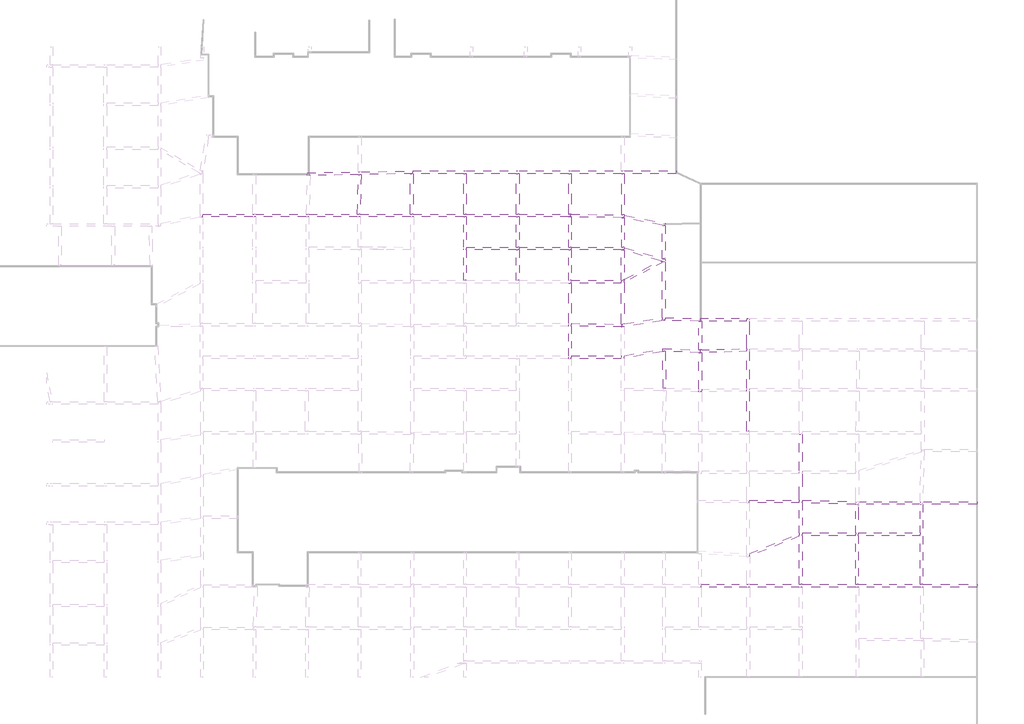
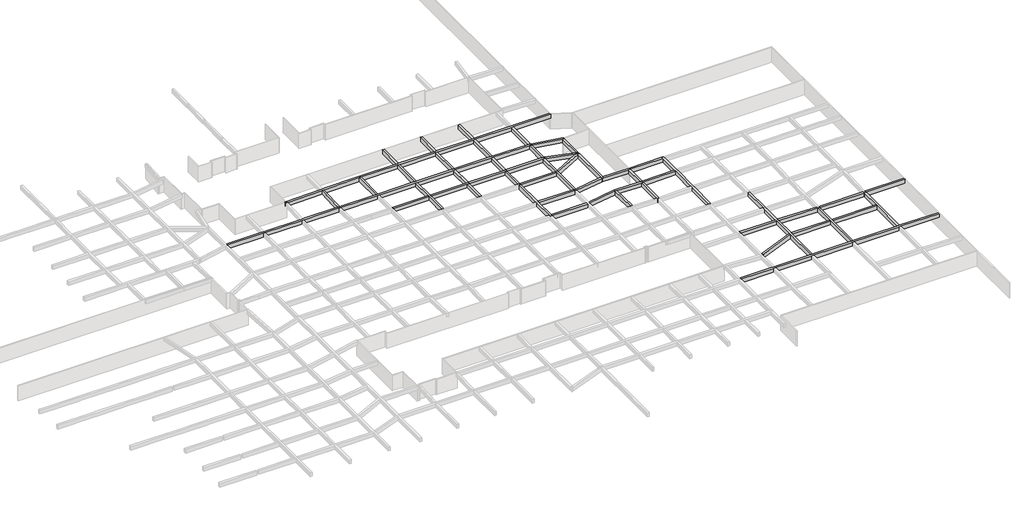
# One storey, part 15 of 20: 51 beams.
"""IFC4 building model written with IfcOpenShell, lengths in millimetres."""

from ifc_helpers import new_model, si_unit, frame, origin, place, context, project, spatial, polyline, outline, extrude, faceted_brep, element, save

model = new_model("IFC4")

# Units and contexts
model_context = context("Model", 3, world=origin())
ifc_project = project(units=[si_unit("LENGTHUNIT", "METRE", prefix="MILLI")], contexts=[model_context])

# Site, building, storey
site = spatial("IfcSite", under=ifc_project)
building = spatial("IfcBuilding", under=site)
storey = spatial("IfcBuildingStorey", under=building, Name="户型图", Elevation=0.0)

# Beams
placement = place(None, origin())
element("IfcBeam", 1, ObjectType="混凝土 - 矩形梁 : KL_beam", at=placement, inside=storey, context=model_context, shape_type="Brep", body=[
    faceted_brep([(163551.2819986, 121489.0, 3300.0), (163350.0, 121489.0, 3300.0), (155979.0, 121489.0, 3300.0), (155579.0, 121489.0, 3300.0), (148179.0, 121489.0, 3300.0), (147779.0, 121489.0, 3300.0), (140279.0, 121489.0, 3300.0), (139879.0, 121489.0, 3300.0), (132410.6079231, 121489.0, 3300.0), (132010.4871741, 121489.0, 3300.0), (124824.0062575, 121489.0, 3300.0), (124423.8311409, 121489.0, 3300.0), (116899.0161386, 121489.0, 3300.0), (116499.0161386, 121489.0, 3300.0), (109085.3829072, 121489.0, 3300.0), (109085.3829072, 121128.9007984, 3300.0), (108907.5439108, 121089.0, 3300.0), (109085.3829072, 121089.0, 3300.0), (116499.0161386, 121089.0, 3300.0), (116899.0161386, 121089.0, 3300.0), (124418.0, 121089.0, 3300.0), (124818.0, 121089.0, 3300.0), (132012.4951791, 121089.0, 3300.0), (132412.7389969, 121089.0, 3300.0), (139950.0, 121089.0, 3300.0), (140350.0, 121089.0, 3300.0), (147750.0, 121089.0, 3300.0), (148150.0, 121089.0, 3300.0), (155579.0, 121089.0, 3300.0), (155979.0, 121089.0, 3300.0), (163350.0, 121089.0, 3300.0), (163548.7180014, 121089.0, 3300.0), (108907.5439108, 121089.0, 2500.0), (109085.3829072, 121089.0, 2500.0), (116499.0161386, 121089.0, 2500.0), (116899.0161386, 121089.0, 2500.0), (124418.0, 121089.0, 2500.0), (124818.0, 121089.0, 2500.0), (132012.4951791, 121089.0, 2500.0), (132412.7389969, 121089.0, 2500.0), (139950.0, 121089.0, 2500.0), (140350.0, 121089.0, 2500.0), (147750.0, 121089.0, 2500.0), (148150.0, 121089.0, 2500.0), (155579.0, 121089.0, 2500.0), (155979.0, 121089.0, 2500.0), (163350.0, 121089.0, 2500.0), (163548.7180014, 121089.0, 2500.0), (109085.3829072, 121128.9007984, 2500.0), (109085.3829072, 121489.0, 2500.0), (116499.0161386, 121489.0, 2500.0), (116899.0161386, 121489.0, 2500.0), (124423.8311409, 121489.0, 2500.0), (124824.0062575, 121489.0, 2500.0), (132010.4871741, 121489.0, 2500.0), (132410.6079231, 121489.0, 2500.0), (139879.0, 121489.0, 2500.0), (140279.0, 121489.0, 2500.0), (147779.0, 121489.0, 2500.0), (148179.0, 121489.0, 2500.0), (155579.0, 121489.0, 2500.0), (155979.0, 121489.0, 2500.0), (163350.0, 121489.0, 2500.0), (163551.2819986, 121489.0, 2500.0)], [[[0, 1, 2, 3, 4, 5, 6, 7, 8, 9, 10, 11, 12, 13, 14, 15, 16, 17, 18, 19, 20, 21, 22, 23, 24, 25, 26, 27, 28, 29, 30, 31]], [[31, 30, 29, 28, 27, 26, 25, 24, 23, 22, 21, 20, 19, 18, 17, 16, 32, 33, 34, 35, 36, 37, 38, 39, 40, 41, 42, 43, 44, 45, 46, 47]], [[47, 46, 45, 44, 43, 42, 41, 40, 39, 38, 37, 36, 35, 34, 33, 32, 48, 49, 50, 51, 52, 53, 54, 55, 56, 57, 58, 59, 60, 61, 62, 63]], [[14, 13, 12, 11, 10, 9, 8, 7, 6, 5, 4, 3, 2, 1, 0, 63, 62, 61, 60, 59, 58, 57, 56, 55, 54, 53, 52, 51, 50, 49]], [[48, 15, 14, 49]], [[15, 48, 32, 16]], [[0, 31, 47, 63]]]),
])
element("IfcBeam", 2, ObjectType="混凝土 - 矩形梁 : KL_beam", at=placement, inside=storey, context=model_context, shape_type="Brep", body=[
    faceted_brep([(171580.0, 121386.0677179, 3300.0), (171180.0, 121391.1959231, 3300.0), (163750.0, 121486.4523333, 3300.0), (163551.2819986, 121489.0, 3300.0), (163548.7180014, 121089.0, 3300.0), (163750.0, 121086.4194616, 3300.0), (171180.0, 120991.1630513, 3300.0), (171359.4728614, 120988.8621172, 3300.0), (171574.8722163, 120986.100587, 3300.0), (163548.7180014, 121089.0, 2500.0), (163750.0, 121086.4194616, 2500.0), (171180.0, 120991.1630513, 2500.0), (171359.4728614, 120988.8621172, 2500.0), (171574.8722163, 120986.100587, 2500.0), (163551.2819986, 121489.0, 2500.0), (163750.0, 121486.4523333, 2500.0), (171180.0, 121391.1959231, 2500.0), (171580.0, 121386.0677179, 2500.0)], [[[0, 1, 2, 3, 4, 5, 6, 7, 8]], [[8, 7, 6, 5, 4, 9, 10, 11, 12, 13]], [[13, 12, 11, 10, 9, 14, 15, 16, 17]], [[3, 2, 1, 0, 17, 16, 15, 14]], [[3, 14, 9, 4]], [[0, 8, 13, 17]]]),
])
element("IfcBeam", 3, ObjectType="混凝土 - 矩形梁 : KL_beam", at=placement, inside=storey, context=model_context, shape_type="Brep", body=[
    faceted_brep([(140199.399879, 127507.7670591, 3300.0), (140195.9091319, 127907.7670591, 3300.0), (132560.0, 127774.4817695, 3300.0), (132160.0, 127767.4997435, 3300.0), (124605.7316919, 127635.6394997, 3300.0), (124593.8863716, 127235.3718076, 3300.0), (124994.2683081, 127242.3605003, 3300.0), (132154.9363056, 127367.3504251, 3300.0), (132555.2287498, 127374.3375558, 3300.0), (140199.399879, 127507.7670591, 2500.0), (124593.8863716, 127235.3718076, 2500.0), (124994.2683081, 127242.3605003, 2500.0), (132154.9363056, 127367.3504251, 2500.0), (132555.2287498, 127374.3375558, 2500.0), (140195.9091319, 127907.7670591, 2500.0), (124605.7316919, 127635.6394997, 2500.0), (132160.0, 127767.4997435, 2500.0), (132560.0, 127774.4817695, 2500.0)], [[[0, 1, 2, 3, 4, 5, 6, 7, 8]], [[9, 0, 8, 7, 6, 5, 10, 11, 12, 13]], [[14, 9, 13, 12, 11, 10, 15, 16, 17]], [[1, 14, 17, 16, 15, 4, 3, 2]], [[1, 0, 9, 14]], [[5, 4, 15, 10]]]),
])
element("IfcBeam", 4, ObjectType="混凝土 - 矩形梁 : KL_beam", at=placement, inside=storey, context=model_context, shape_type="Brep", body=[
    faceted_brep([(179299.7116785, 127907.7670591, 3300.0), (179299.7116785, 127507.7670591, 3300.0), (179299.7116785, 127507.7670591, 2500.0), (179299.7116785, 127907.7670591, 2500.0), (171549.0, 127907.7670591, 3300.0), (171149.0, 127907.7670591, 3300.0), (163750.0, 127907.7670591, 3300.0), (163350.0, 127907.7670591, 3300.0), (155979.0, 127907.7670591, 3300.0), (155579.0, 127907.7670591, 3300.0), (148179.0, 127907.7670591, 3300.0), (147779.0, 127907.7670591, 3300.0), (140195.9091319, 127907.7670591, 3300.0), (140199.399879, 127507.7670591, 3300.0), (147779.0, 127507.7670591, 3300.0), (148179.0, 127507.7670591, 3300.0), (155579.0, 127507.7670591, 3300.0), (155979.0, 127507.7670591, 3300.0), (163350.0, 127507.7670591, 3300.0), (163750.0, 127507.7670591, 3300.0), (171180.0, 127507.7670591, 3300.0), (171580.0, 127507.7670591, 3300.0), (140199.399879, 127507.7670591, 2500.0), (147779.0, 127507.7670591, 2500.0), (148179.0, 127507.7670591, 2500.0), (155579.0, 127507.7670591, 2500.0), (155979.0, 127507.7670591, 2500.0), (163350.0, 127507.7670591, 2500.0), (163750.0, 127507.7670591, 2500.0), (171180.0, 127507.7670591, 2500.0), (171580.0, 127507.7670591, 2500.0), (140195.9091319, 127907.7670591, 2500.0), (147779.0, 127907.7670591, 2500.0), (148179.0, 127907.7670591, 2500.0), (155579.0, 127907.7670591, 2500.0), (155979.0, 127907.7670591, 2500.0), (163350.0, 127907.7670591, 2500.0), (163750.0, 127907.7670591, 2500.0), (171149.0, 127907.7670591, 2500.0), (171549.0, 127907.7670591, 2500.0)], [[[0, 1, 2, 3]], [[1, 0, 4, 5, 6, 7, 8, 9, 10, 11, 12, 13, 14, 15, 16, 17, 18, 19, 20, 21]], [[2, 1, 21, 20, 19, 18, 17, 16, 15, 14, 13, 22, 23, 24, 25, 26, 27, 28, 29, 30]], [[3, 2, 30, 29, 28, 27, 26, 25, 24, 23, 22, 31, 32, 33, 34, 35, 36, 37, 38, 39]], [[0, 3, 39, 38, 37, 36, 35, 34, 33, 32, 31, 12, 11, 10, 9, 8, 7, 6, 5, 4]], [[12, 31, 22, 13]]]),
])
element("IfcBeam", 5, ObjectType="混凝土 - 矩形梁 : KL_beam", at=placement, inside=storey, context=model_context, shape_type="SweptSolid", body=[
    extrude(outline(polyline([(163350.0, 132993.0), (163750.0, 132993.0), (163750.0, 127907.7670591), (163350.0, 127907.7670591), (163350.0, 132993.0)])), frame((0.0, 0.0, 2500.0), z_axis=(0.0, 0.0, 1.0), x_axis=(1.0, 0.0, 0.0)), (0.0, 0.0, 1.0), 800.0),
    extrude(outline(polyline([(163551.2819986, 121489.0), (163350.0, 121489.0), (163350.0, 127507.7670591), (163750.0, 127507.7670591), (163750.0, 121486.4523333), (163551.2819986, 121489.0)])), frame((0.0, 0.0, 2500.0), z_axis=(0.0, 0.0, 1.0), x_axis=(1.0, 0.0, 0.0)), (0.0, 0.0, 1.0), 800.0),
])
element("IfcBeam", 6, ObjectType="混凝土 - 矩形梁 : KL_beam", at=placement, inside=storey, context=model_context, shape_type="SweptSolid", body=[
    extrude(outline(polyline([(155579.0, 132993.0), (155979.0, 132993.0), (155979.0, 127907.7670591), (155579.0, 127907.7670591), (155579.0, 132993.0)])), frame((0.0, 0.0, 2500.0), z_axis=(0.0, 0.0, 1.0), x_axis=(1.0, 0.0, 0.0)), (0.0, 0.0, 1.0), 800.0),
    extrude(outline(polyline([(155979.0, 121489.0), (155579.0, 121489.0), (155579.0, 127507.7670591), (155979.0, 127507.7670591), (155979.0, 121489.0)])), frame((0.0, 0.0, 2500.0), z_axis=(0.0, 0.0, 1.0), x_axis=(1.0, 0.0, 0.0)), (0.0, 0.0, 1.0), 800.0),
])
element("IfcBeam", 7, ObjectType="混凝土 - 矩形梁 : KL_beam", at=placement, inside=storey, context=model_context, shape_type="SweptSolid", body=[
    extrude(outline(polyline([(147779.0, 132995.0), (148179.0, 132995.0), (148179.0, 127907.7670591), (147779.0, 127907.7670591), (147779.0, 132995.0)])), frame((0.0, 0.0, 2500.0), z_axis=(0.0, 0.0, 1.0), x_axis=(1.0, 0.0, 0.0)), (0.0, 0.0, 1.0), 800.0),
    extrude(outline(polyline([(148179.0, 121489.0), (147779.0, 121489.0), (147779.0, 127507.7670591), (148179.0, 127507.7670591), (148179.0, 121489.0)])), frame((0.0, 0.0, 2500.0), z_axis=(0.0, 0.0, 1.0), x_axis=(1.0, 0.0, 0.0)), (0.0, 0.0, 1.0), 800.0),
])
element("IfcBeam", 8, ObjectType="混凝土 - 矩形梁 : KL_beam", at=placement, inside=storey, context=model_context, shape_type="SweptSolid", body=[
    extrude(outline(polyline([(139879.0, 127488.6479685), (140279.0, 127488.6479685), (140279.0, 121489.0), (139879.0, 121489.0), (139879.0, 127488.6479685)])), frame((0.0, 0.0, 2500.0), z_axis=(0.0, 0.0, 1.0), x_axis=(1.0, 0.0, 0.0)), (0.0, 0.0, 1.0), 800.0),
])
element("IfcBeam", 9, ObjectType="混凝土 - 矩形梁 : KL_beam", at=placement, inside=storey, context=model_context, shape_type="Brep", body=[
    faceted_brep([(171574.8722163, 120986.100587, 3300.0), (171580.0, 120986.0348462, 3300.0), (171580.0, 121353.4826618, 3300.0), (171580.0, 121386.0677179, 3300.0), (171180.0, 121391.1959231, 2500.0), (171180.0, 121391.1959231, 3300.0), (171180.0, 127507.7670591, 3300.0), (171180.0, 127507.7670591, 2500.0), (171580.0, 120986.0348462, 2500.0), (171574.8722163, 120986.100587, 2500.0), (171580.0, 121386.0677179, 2500.0), (171580.0, 121353.4826618, 2500.0), (171580.0, 127507.7670591, 2500.0), (171580.0, 127507.7670591, 3300.0)], [[[0, 1, 2, 3]], [[4, 5, 6, 7]], [[8, 9, 10, 11]], [[1, 8, 11, 10, 12, 13, 3, 2]], [[8, 1, 0, 9]], [[10, 3, 5, 4]], [[3, 10, 9, 0]], [[5, 3, 13, 6]], [[10, 4, 7, 12]], [[7, 6, 13, 12]]]),
])
element("IfcBeam", 10, ObjectType="混凝土 - 矩形梁 : KL_beam", at=placement, inside=storey, context=model_context, shape_type="Brep", body=[
    faceted_brep([(171580.0, 120986.0348462, 3300.0), (171574.8722163, 120986.100587, 3300.0), (171359.4728614, 120988.8621172, 3300.0), (171580.0, 120945.9959838, 3300.0), (177250.0, 119843.859631, 3300.0), (177650.0, 119766.1075073, 3300.0), (177650.0, 120173.5941853, 3300.0), (171580.0, 121353.4826618, 3300.0), (171359.4728614, 120988.8621172, 2500.0), (171580.0, 120945.9959838, 2500.0), (177250.0, 119843.859631, 2500.0), (177650.0, 119766.1075073, 2500.0), (171574.8722163, 120986.100587, 2500.0), (171580.0, 120986.0348462, 2500.0), (171580.0, 121353.4826618, 2500.0), (177650.0, 120173.5941853, 2500.0)], [[[0, 1, 2, 3, 4, 5, 6, 7]], [[2, 8, 9, 10, 11, 5, 4, 3]], [[8, 12, 13, 14, 15, 11, 10, 9]], [[6, 15, 14, 7]], [[0, 13, 12, 8, 2, 1]], [[13, 0, 7, 14]], [[6, 5, 11, 15]]]),
])
element("IfcBeam", 11, ObjectType="混凝土 - 矩形梁 : KL_beam", at=placement, inside=storey, context=model_context, shape_type="SweptSolid", body=[
    extrude(outline(polyline([(132410.6079231, 121489.0), (132010.4871741, 121489.0), (132154.9363056, 127367.3504251), (132555.2287498, 127374.3375558), (132410.6079231, 121489.0)])), frame((0.0, 0.0, 2500.0), z_axis=(0.0, 0.0, 1.0), x_axis=(1.0, 0.0, 0.0)), (0.0, 0.0, 1.0), 800.0),
])
element("IfcBeam", 12, ObjectType="混凝土 - 矩形梁 : KL_beam", at=placement, inside=storey, context=model_context, shape_type="Brep", body=[
    faceted_brep([(223898.0, 66590.0, 3300.0), (223898.0, 66190.0, 3300.0), (223898.0, 66190.0, 2500.0), (223898.0, 66590.0, 2500.0), (215847.0, 66590.0, 3300.0), (215447.0, 66590.0, 3300.0), (206300.0, 66590.0, 3300.0), (205900.0, 66590.0, 3300.0), (197962.0, 66590.0, 3300.0), (197562.0, 66590.0, 3300.0), (190162.0, 66590.0, 3300.0), (189762.0, 66590.0, 3300.0), (183030.0, 66590.0, 3300.0), (183030.0, 66190.0, 3300.0), (189762.0, 66190.0, 3300.0), (190162.0, 66190.0, 3300.0), (197562.0, 66190.0, 3300.0), (197962.0, 66190.0, 3300.0), (205962.0, 66190.0, 3300.0), (206362.0, 66190.0, 3300.0), (215538.0, 66190.0, 3300.0), (215938.0, 66190.0, 3300.0), (183030.0, 66190.0, 2500.0), (189762.0, 66190.0, 2500.0), (190162.0, 66190.0, 2500.0), (197562.0, 66190.0, 2500.0), (197962.0, 66190.0, 2500.0), (205962.0, 66190.0, 2500.0), (206362.0, 66190.0, 2500.0), (215538.0, 66190.0, 2500.0), (215938.0, 66190.0, 2500.0), (183030.0, 66590.0, 2500.0), (189762.0, 66590.0, 2500.0), (190162.0, 66590.0, 2500.0), (197562.0, 66590.0, 2500.0), (197962.0, 66590.0, 2500.0), (205900.0, 66590.0, 2500.0), (206300.0, 66590.0, 2500.0), (215447.0, 66590.0, 2500.0), (215847.0, 66590.0, 2500.0)], [[[0, 1, 2, 3]], [[1, 0, 4, 5, 6, 7, 8, 9, 10, 11, 12, 13, 14, 15, 16, 17, 18, 19, 20, 21]], [[2, 1, 21, 20, 19, 18, 17, 16, 15, 14, 13, 22, 23, 24, 25, 26, 27, 28, 29, 30]], [[3, 2, 30, 29, 28, 27, 26, 25, 24, 23, 22, 31, 32, 33, 34, 35, 36, 37, 38, 39]], [[0, 3, 39, 38, 37, 36, 35, 34, 33, 32, 31, 12, 11, 10, 9, 8, 7, 6, 5, 4]], [[13, 12, 31, 22]]]),
])
element("IfcBeam", 13, ObjectType="混凝土 - 矩形梁 : KL_beam", at=placement, inside=storey, context=model_context, shape_type="Brep", body=[
    faceted_brep([(148150.0, 121089.0, 3300.0), (147750.0, 121089.0, 3300.0), (147750.0, 116589.0, 3300.0), (147750.0, 116189.0, 3300.0), (147750.0, 111689.0, 3300.0), (148150.0, 111689.0, 3300.0), (148150.0, 116189.0, 3300.0), (148150.0, 116589.0, 3300.0), (148150.0, 121089.0, 2500.0), (148150.0, 111689.0, 2500.0), (148150.0, 116189.0, 2500.0), (148150.0, 116589.0, 2500.0), (147750.0, 121089.0, 2500.0), (147750.0, 111689.0, 2500.0), (147750.0, 116189.0, 2500.0), (147750.0, 116589.0, 2500.0)], [[[0, 1, 2, 3, 4, 5, 6, 7]], [[8, 0, 7, 6, 5, 9, 10, 11]], [[12, 8, 11, 10, 9, 13, 14, 15]], [[1, 12, 15, 14, 13, 4, 3, 2]], [[1, 0, 8, 12]], [[5, 4, 13, 9]]]),
])
element("IfcBeam", 14, ObjectType="混凝土 - 矩形梁 : KL_beam", at=placement, inside=storey, context=model_context, shape_type="Brep", body=[
    faceted_brep([(140350.0, 116589.0, 3300.0), (140350.0, 116189.0, 3300.0), (147750.0, 116189.0, 3300.0), (147750.0, 116589.0, 3300.0), (140350.0, 116189.0, 2500.0), (147750.0, 116189.0, 2500.0), (140350.0, 116589.0, 2500.0), (147750.0, 116589.0, 2500.0)], [[[0, 1, 2, 3]], [[1, 4, 5, 2]], [[4, 6, 7, 5]], [[6, 0, 3, 7]], [[1, 0, 6, 4]], [[3, 2, 5, 7]]]),
    faceted_brep([(148150.0, 116189.0, 3300.0), (148150.0, 116589.0, 3300.0), (148150.0, 116589.0, 2500.0), (148150.0, 116189.0, 2500.0), (155979.0, 116189.0, 3300.0), (155979.0, 116589.0, 3300.0), (155579.0, 116589.0, 3300.0), (155579.0, 116189.0, 3300.0), (155979.0, 116189.0, 2500.0), (155579.0, 116189.0, 2500.0), (155979.0, 116589.0, 2500.0), (155579.0, 116589.0, 2500.0)], [[[0, 1, 2, 3]], [[4, 5, 6, 1, 0, 7]], [[8, 4, 7, 0, 3, 9]], [[10, 8, 9, 3, 2, 11]], [[5, 10, 11, 2, 1, 6]], [[5, 4, 8, 10]]]),
])
element("IfcBeam", 15, ObjectType="混凝土 - 矩形梁 : KL_beam", at=placement, inside=storey, context=model_context, shape_type="SweptSolid", body=[
    extrude(outline(polyline([(155979.0, 116589.0), (155579.0, 116589.0), (155579.0, 121089.0), (155979.0, 121089.0), (155979.0, 116589.0)])), frame((0.0, 0.0, 2500.0), z_axis=(0.0, 0.0, 1.0), x_axis=(1.0, 0.0, 0.0)), (0.0, 0.0, 1.0), 800.0),
])
element("IfcBeam", 16, ObjectType="混凝土 - 矩形梁 : KL_beam", at=placement, inside=storey, context=model_context, shape_type="SweptSolid", body=[
    extrude(outline(polyline([(155579.0, 116189.0), (155979.0, 116189.0), (155979.0, 111689.0), (155579.0, 111689.0), (155579.0, 116189.0)])), frame((0.0, 0.0, 2500.0), z_axis=(0.0, 0.0, 1.0), x_axis=(1.0, 0.0, 0.0)), (0.0, 0.0, 1.0), 800.0),
])
element("IfcBeam", 17, ObjectType="混凝土 - 矩形梁 : KL_beam", at=placement, inside=storey, context=model_context, shape_type="Brep", body=[
    faceted_brep([(163750.0, 116189.0, 3300.0), (163750.0, 116589.0, 3300.0), (163350.0, 116589.0, 3300.0), (155979.0, 116589.0, 3300.0), (155979.0, 116189.0, 3300.0), (163350.0, 116189.0, 3300.0), (163750.0, 116189.0, 2500.0), (155979.0, 116189.0, 2500.0), (163350.0, 116189.0, 2500.0), (163750.0, 116589.0, 2500.0), (155979.0, 116589.0, 2500.0), (163350.0, 116589.0, 2500.0)], [[[0, 1, 2, 3, 4, 5]], [[6, 0, 5, 4, 7, 8]], [[9, 6, 8, 7, 10, 11]], [[1, 9, 11, 10, 3, 2]], [[4, 3, 10, 7]], [[1, 0, 6, 9]]]),
])
element("IfcBeam", 18, ObjectType="混凝土 - 矩形梁 : KL_beam", at=placement, inside=storey, context=model_context, shape_type="SweptSolid", body=[
    extrude(outline(polyline([(163350.0, 121089.0), (163548.7180014, 121089.0), (163750.0, 121086.4194616), (163750.0, 116589.0), (163350.0, 116589.0), (163350.0, 121089.0)])), frame((0.0, 0.0, 2500.0), z_axis=(0.0, 0.0, 1.0), x_axis=(1.0, 0.0, 0.0)), (0.0, 0.0, 1.0), 800.0),
])
element("IfcBeam", 19, ObjectType="混凝土 - 矩形梁 : KL_beam", at=placement, inside=storey, context=model_context, shape_type="SweptSolid", body=[
    extrude(outline(polyline([(163350.0, 116189.0), (163750.0, 116189.0), (163750.0, 111689.0), (163350.0, 111689.0), (163350.0, 116189.0)])), frame((0.0, 0.0, 2500.0), z_axis=(0.0, 0.0, 1.0), x_axis=(1.0, 0.0, 0.0)), (0.0, 0.0, 1.0), 800.0),
])
element("IfcBeam", 20, ObjectType="混凝土 - 矩形梁 : KL_beam", at=placement, inside=storey, context=model_context, shape_type="Brep", body=[
    faceted_brep([(171580.0, 116189.0, 3300.0), (171580.0, 116539.71081, 3300.0), (171580.0, 116589.0, 3300.0), (171180.0, 116589.0, 3300.0), (163750.0, 116589.0, 3300.0), (163750.0, 116189.0, 3300.0), (171150.0, 116189.0, 3300.0), (171351.8918331, 116189.0, 3300.0), (171580.0, 116189.0, 2500.0), (163750.0, 116189.0, 2500.0), (171150.0, 116189.0, 2500.0), (171351.8918331, 116189.0, 2500.0), (171580.0, 116589.0, 2500.0), (171580.0, 116539.71081, 2500.0), (163750.0, 116589.0, 2500.0), (171180.0, 116589.0, 2500.0)], [[[0, 1, 2, 3, 4, 5, 6, 7]], [[8, 0, 7, 6, 5, 9, 10, 11]], [[12, 13, 8, 11, 10, 9, 14, 15]], [[2, 12, 15, 14, 4, 3]], [[5, 4, 14, 9]], [[2, 1, 0, 8, 13, 12]]]),
])
element("IfcBeam", 21, ObjectType="混凝土 - 矩形梁 : KL_beam", at=placement, inside=storey, context=model_context, shape_type="SweptSolid", body=[
    extrude(outline(polyline([(171180.0, 120991.1630513), (171359.4728614, 120988.8621172), (171580.0, 120945.9959838), (171580.0, 116589.0), (171180.0, 116589.0), (171180.0, 120991.1630513)])), frame((0.0, 0.0, 2500.0), z_axis=(0.0, 0.0, 1.0), x_axis=(1.0, 0.0, 0.0)), (0.0, 0.0, 1.0), 800.0),
])
element("IfcBeam", 22, ObjectType="混凝土 - 矩形梁 : KL_beam", at=placement, inside=storey, context=model_context, shape_type="Brep", body=[
    faceted_brep([(171580.0, 116189.0, 3300.0), (171351.8918331, 116189.0, 3300.0), (171550.0, 116132.1933972, 3300.0), (176911.537907, 114594.7971419, 3300.0), (177250.0, 114497.7446984, 3300.0), (177650.0, 114383.0465441, 3300.0), (177650.0, 114799.1663185, 3300.0), (177428.6567193, 114862.6354829, 3300.0), (177250.0, 114913.8644728, 3300.0), (171580.0, 116539.71081, 3300.0), (171351.8918331, 116189.0, 2500.0), (171550.0, 116132.1933972, 2500.0), (176911.537907, 114594.7971419, 2500.0), (177250.0, 114497.7446984, 2500.0), (177650.0, 114383.0465441, 2500.0), (171580.0, 116189.0, 2500.0), (171580.0, 116539.71081, 2500.0), (177250.0, 114913.8644728, 2500.0), (177428.6567193, 114862.6354829, 2500.0), (177650.0, 114799.1663185, 2500.0)], [[[0, 1, 2, 3, 4, 5, 6, 7, 8, 9]], [[1, 10, 11, 12, 13, 14, 5, 4, 3, 2]], [[10, 15, 16, 17, 18, 19, 14, 13, 12, 11]], [[16, 9, 8, 7, 6, 19, 18, 17]], [[0, 15, 10, 1]], [[15, 0, 9, 16]], [[6, 5, 14, 19]]]),
])
element("IfcBeam", 23, ObjectType="混凝土 - 矩形梁 : KL_beam", at=placement, inside=storey, context=model_context, shape_type="Brep", body=[
    faceted_brep([(177250.0, 105717.8300868, 3300.0), (177419.9721071, 105744.7510238, 3300.0), (177650.0, 105781.1838629, 3300.0), (177650.0, 106140.7968032, 3300.0), (177650.0, 114383.0465441, 3300.0), (177250.0, 114497.7446984, 3300.0), (177250.0, 114319.6322148, 3300.0), (177250.0, 106122.8161371, 3300.0), (177250.0, 105717.8300868, 2500.0), (177250.0, 114497.7446984, 2500.0), (177250.0, 114319.6322148, 2500.0), (177250.0, 106122.8161371, 2500.0), (177650.0, 105781.1838629, 2500.0), (177419.9721071, 105744.7510238, 2500.0), (177650.0, 114383.0465441, 2500.0), (177650.0, 106140.7968032, 2500.0)], [[[0, 1, 2, 3, 4, 5, 6, 7]], [[8, 0, 7, 6, 5, 9, 10, 11]], [[12, 13, 8, 11, 10, 9, 14, 15]], [[2, 12, 15, 14, 4, 3]], [[5, 4, 14, 9]], [[2, 1, 0, 8, 13, 12]]]),
])
element("IfcBeam", 24, ObjectType="混凝土 - 矩形梁 : KL_beam", at=placement, inside=storey, context=model_context, shape_type="Brep", body=[
    faceted_brep([(171150.0, 105156.6710511, 3300.0), (171208.4377833, 104787.7094085, 3300.0), (171212.573786, 104761.5957149, 3300.0), (171364.4255325, 104785.6466688, 3300.0), (171550.0, 104815.0387769, 3300.0), (177250.0, 105717.8300868, 3300.0), (177250.0, 106122.8161371, 3300.0), (171550.0, 105220.0248272, 3300.0), (171150.0, 105156.6710511, 2500.0), (177250.0, 106122.8161371, 2500.0), (171550.0, 105220.0248272, 2500.0), (171212.573786, 104761.5957149, 2500.0), (171208.4377833, 104787.7094085, 2500.0), (177250.0, 105717.8300868, 2500.0), (171550.0, 104815.0387769, 2500.0), (171364.4255325, 104785.6466688, 2500.0)], [[[0, 1, 2, 3, 4, 5, 6, 7]], [[8, 0, 7, 6, 9, 10]], [[11, 12, 8, 10, 9, 13, 14, 15]], [[2, 11, 15, 14, 13, 5, 4, 3]], [[6, 5, 13, 9]], [[2, 1, 0, 8, 12, 11]]]),
])
element("IfcBeam", 25, ObjectType="混凝土 - 矩形梁 : KL_beam", at=placement, inside=storey, context=model_context, shape_type="Brep", body=[
    faceted_brep([(171550.0, 111817.8232937, 3300.0), (171150.0, 111610.6458833, 3300.0), (171150.0, 111289.0, 3300.0), (171150.0, 105188.5171458, 3300.0), (171150.0, 105156.6710511, 3300.0), (171550.0, 105220.0248272, 3300.0), (171550.0, 111367.3541167, 3300.0), (171150.0, 111610.6458833, 2500.0), (171150.0, 111289.0, 2500.0), (171150.0, 105188.5171458, 2500.0), (171150.0, 105156.6710511, 2500.0), (171550.0, 111817.8232937, 2500.0), (171550.0, 111367.3541167, 2500.0), (171550.0, 105220.0248272, 2500.0)], [[[0, 1, 2, 3, 4, 5, 6]], [[1, 7, 8, 9, 10, 4, 3, 2]], [[7, 11, 12, 13, 10, 9, 8]], [[11, 0, 6, 5, 13, 12]], [[5, 4, 10, 13]], [[1, 0, 11, 7]]]),
])
element("IfcBeam", 26, ObjectType="混凝土 - 矩形梁 : KL_beam", at=placement, inside=storey, context=model_context, shape_type="Brep", body=[
    faceted_brep([(171351.8918331, 116189.0, 3300.0), (171150.0, 116189.0, 3300.0), (171150.0, 111689.0, 3300.0), (171150.0, 111610.6458833, 3300.0), (171550.0, 111817.8232937, 3300.0), (171550.0, 116132.1933972, 3300.0), (171550.0, 116132.1933972, 2500.0), (171550.0, 111817.8232937, 2500.0), (171150.0, 116189.0, 2500.0), (171351.8918331, 116189.0, 2500.0), (171150.0, 111610.6458833, 2500.0), (171150.0, 111689.0, 2500.0)], [[[0, 1, 2, 3, 4, 5]], [[6, 5, 4, 7]], [[8, 9, 6, 7, 10, 11]], [[1, 8, 11, 10, 3, 2]], [[8, 1, 0, 9]], [[0, 5, 6, 9]], [[4, 3, 10, 7]]]),
])
element("IfcBeam", 27, ObjectType="混凝土 - 矩形梁 : KL_beam", at=placement, inside=storey, context=model_context, shape_type="SweptSolid", body=[
    extrude(outline(polyline([(177650.0, 114799.1663185), (177428.6567193, 114862.6354829), (177650.0, 114977.2788021), (177650.0, 114799.1663185)])), frame((0.0, 0.0, 2500.0), z_axis=(0.0, 0.0, 1.0), x_axis=(1.0, 0.0, 0.0)), (0.0, 0.0, 1.0), 800.0),
    extrude(outline(polyline([(176911.537907, 114594.7971419), (177250.0, 114497.7446984), (177250.0, 114319.6322148), (171550.0, 111367.3541167), (171550.0, 111817.8232937), (176911.537907, 114594.7971419)])), frame((0.0, 0.0, 2500.0), z_axis=(0.0, 0.0, 1.0), x_axis=(1.0, 0.0, 0.0)), (0.0, 0.0, 1.0), 800.0),
])
element("IfcBeam", 28, ObjectType="混凝土 - 矩形梁 : KL_beam", at=placement, inside=storey, context=model_context, shape_type="Brep", body=[
    faceted_brep([(163750.0, 111689.0, 3300.0), (163750.0, 111289.0, 3300.0), (171150.0, 111289.0, 3300.0), (171150.0, 111610.6458833, 3300.0), (171150.0, 111689.0, 3300.0), (163750.0, 111289.0, 2500.0), (171150.0, 111289.0, 2500.0), (163750.0, 111689.0, 2500.0), (171150.0, 111689.0, 2500.0), (171150.0, 111610.6458833, 2500.0)], [[[0, 1, 2, 3, 4]], [[1, 5, 6, 2]], [[5, 7, 8, 9, 6]], [[7, 0, 4, 8]], [[1, 0, 7, 5]], [[2, 6, 9, 8, 4, 3]]]),
])
element("IfcBeam", 29, ObjectType="混凝土 - 矩形梁 : KL_beam", at=placement, inside=storey, context=model_context, shape_type="Brep", body=[
    faceted_brep([(171208.4377833, 104787.7094085, 3300.0), (171150.0, 105156.6710511, 3300.0), (171150.0, 105188.5171458, 3300.0), (163750.0, 105286.3727401, 3300.0), (163750.0, 104886.3377683, 3300.0), (171150.0, 104788.4821739, 3300.0), (171150.0, 105188.5171458, 2500.0), (163750.0, 105286.3727401, 2500.0), (171150.0, 105156.6710511, 2500.0), (171208.4377833, 104787.7094085, 2500.0), (171150.0, 104788.4821739, 2500.0), (163750.0, 104886.3377683, 2500.0)], [[[0, 1, 2, 3, 4, 5]], [[2, 6, 7, 3]], [[8, 9, 10, 11, 7, 6]], [[9, 0, 5, 4, 11, 10]], [[1, 0, 9, 8]], [[2, 1, 8, 6]], [[4, 3, 7, 11]]]),
    faceted_brep([(171550.0, 104815.0387769, 2500.0), (171550.0, 104815.0387769, 3300.0), (171550.0, 104783.1926823, 3300.0), (171550.0, 104783.1926823, 2500.0), (171364.4255325, 104785.6466688, 3300.0), (171364.4255325, 104785.6466688, 2500.0)], [[[0, 1, 2, 3]], [[4, 1, 0, 5]], [[1, 4, 2]], [[5, 0, 3]], [[4, 5, 3, 2]]]),
])
element("IfcBeam", 30, ObjectType="混凝土 - 矩形梁 : KL_beam", at=placement, inside=storey, context=model_context, shape_type="Brep", body=[
    faceted_brep([(163350.0, 100089.0, 3300.0), (163750.0, 100089.0, 3300.0), (163750.0, 100489.0, 3300.0), (163750.0, 104886.3377683, 3300.0), (163750.0, 105286.3727401, 3300.0), (163750.0, 111289.0, 3300.0), (163350.0, 111289.0, 3300.0), (163350.0, 105289.0, 3300.0), (163350.0, 104889.0, 3300.0), (163350.0, 100489.0, 3300.0), (163350.0, 100089.0, 2500.0), (163350.0, 111289.0, 2500.0), (163350.0, 105289.0, 2500.0), (163350.0, 104889.0, 2500.0), (163350.0, 100489.0, 2500.0), (163750.0, 100089.0, 2500.0), (163750.0, 111289.0, 2500.0), (163750.0, 105286.3727401, 2500.0), (163750.0, 104886.3377683, 2500.0), (163750.0, 100489.0, 2500.0)], [[[0, 1, 2, 3, 4, 5, 6, 7, 8, 9]], [[10, 0, 9, 8, 7, 6, 11, 12, 13, 14]], [[15, 10, 14, 13, 12, 11, 16, 17, 18, 19]], [[1, 15, 19, 18, 17, 16, 5, 4, 3, 2]], [[6, 5, 16, 11]], [[1, 0, 10, 15]]]),
])
element("IfcBeam", 31, ObjectType="混凝土 - 矩形梁 : KL_beam", at=placement, inside=storey, context=model_context, shape_type="SweptSolid", body=[
    extrude(outline(polyline([(163750.0, 100089.0), (163750.0, 100489.0), (171150.0, 100489.0), (171150.0, 100089.0), (163750.0, 100089.0)])), frame((0.0, 0.0, 2500.0), z_axis=(0.0, 0.0, 1.0), x_axis=(1.0, 0.0, 0.0)), (0.0, 0.0, 1.0), 800.0),
])
element("IfcBeam", 32, ObjectType="混凝土 - 矩形梁 : KL_beam", at=placement, inside=storey, context=model_context, shape_type="Brep", body=[
    faceted_brep([(190150.0341333, 106050.0, 3300.0), (189750.0341333, 106050.0, 3300.0), (189750.0341333, 105650.0, 3300.0), (189750.0341333, 101545.5545912, 3300.0), (189750.0341333, 101145.4202286, 3300.0), (189750.0341333, 95660.4589312, 3300.0), (189750.0341333, 95260.398, 3300.0), (189750.0341333, 89291.7476257, 3300.0), (190150.0341333, 89291.7476257, 3300.0), (190150.0341333, 95263.9194786, 3300.0), (190150.0341333, 95663.9194786, 3300.0), (190150.0341333, 101150.0, 3300.0), (190150.0341333, 101550.0, 3300.0), (190150.0341333, 105650.0, 3300.0), (190150.0341333, 106050.0, 2500.0), (190150.0341333, 89291.7476257, 2500.0), (190150.0341333, 95263.9194786, 2500.0), (190150.0341333, 95663.9194786, 2500.0), (190150.0341333, 101150.0, 2500.0), (190150.0341333, 101550.0, 2500.0), (190150.0341333, 105650.0, 2500.0), (189750.0341333, 106050.0, 2500.0), (189750.0341333, 89291.7476257, 2500.0), (189750.0341333, 95260.398, 2500.0), (189750.0341333, 95660.4589312, 2500.0), (189750.0341333, 101145.4202286, 2500.0), (189750.0341333, 101545.5545912, 2500.0), (189750.0341333, 105650.0, 2500.0)], [[[0, 1, 2, 3, 4, 5, 6, 7, 8, 9, 10, 11, 12, 13]], [[14, 0, 13, 12, 11, 10, 9, 8, 15, 16, 17, 18, 19, 20]], [[21, 14, 20, 19, 18, 17, 16, 15, 22, 23, 24, 25, 26, 27]], [[1, 21, 27, 26, 25, 24, 23, 22, 7, 6, 5, 4, 3, 2]], [[8, 7, 22, 15]], [[1, 0, 14, 21]]]),
])
element("IfcBeam", 33, ObjectType="混凝土 - 矩形梁 : KL_beam", at=placement, inside=storey, context=model_context, shape_type="Brep", body=[
    faceted_brep([(182851.7453736, 106050.0, 3300.0), (182848.2546264, 105650.0, 3300.0), (183046.7104659, 105650.0, 3300.0), (189750.0341333, 105650.0, 3300.0), (189750.0341333, 106050.0, 3300.0), (182851.7453736, 106050.0, 2500.0), (189750.0341333, 106050.0, 2500.0), (182848.2546264, 105650.0, 2500.0), (189750.0341333, 105650.0, 2500.0), (183046.7104659, 105650.0, 2500.0)], [[[0, 1, 2, 3, 4]], [[5, 0, 4, 6]], [[7, 5, 6, 8, 9]], [[1, 7, 9, 8, 3, 2]], [[4, 3, 8, 6]], [[1, 0, 5, 7]]]),
])
element("IfcBeam", 34, ObjectType="混凝土 - 矩形梁 : KL_beam", at=placement, inside=storey, context=model_context, shape_type="Brep", body=[
    faceted_brep([(182848.2546264, 105650.0, 2500.0), (182848.2546264, 105650.0, 3300.0), (182646.7104659, 105653.5179664, 3300.0), (177419.9721071, 105744.7510238, 3300.0), (177419.9721071, 105744.7510238, 2500.0), (182646.7104659, 105653.5179664, 2500.0), (182851.7453736, 106050.0, 2500.0), (182851.7453736, 106050.0, 3300.0), (177650.0, 105781.1838629, 3300.0), (177650.0, 105781.1838629, 2500.0), (177650.0, 106140.7968032, 3300.0), (177650.0, 106140.7968032, 2500.0)], [[[0, 1, 2, 3, 4, 5]], [[1, 0, 6, 7]], [[8, 9, 4, 3]], [[9, 8, 10, 11]], [[1, 7, 10, 8, 3, 2]], [[7, 6, 11, 10]], [[6, 0, 5, 4, 9, 11]]]),
])
element("IfcBeam", 35, ObjectType="混凝土 - 矩形梁 : KL_beam", at=placement, inside=storey, context=model_context, shape_type="Brep", body=[
    faceted_brep([(182845.8109669, 100966.4522201, 3300.0), (182847.6099649, 101366.6332155, 3300.0), (182646.7104659, 101373.6487806, 3300.0), (177268.0337325, 101561.4763109, 3300.0), (177254.0739338, 101161.7199801, 3300.0), (177654.4627654, 101147.738094, 3300.0), (182646.7104659, 100973.4049628, 3300.0), (182845.8109669, 100966.4522201, 2500.0), (177254.0739338, 101161.7199801, 2500.0), (177654.4627654, 101147.738094, 2500.0), (182646.7104659, 100973.4049628, 2500.0), (182847.6099649, 101366.6332155, 2500.0), (177268.0337325, 101561.4763109, 2500.0), (182646.7104659, 101373.6487806, 2500.0)], [[[0, 1, 2, 3, 4, 5, 6]], [[7, 0, 6, 5, 4, 8, 9, 10]], [[11, 7, 10, 9, 8, 12, 13]], [[1, 11, 13, 12, 3, 2]], [[1, 0, 7, 11]], [[3, 12, 8, 4]]]),
])
element("IfcBeam", 36, ObjectType="混凝土 - 矩形梁 : KL_beam", at=placement, inside=storey, context=model_context, shape_type="Brep", body=[
    faceted_brep([(182847.6099649, 101366.6332155, 3300.0), (182845.8109669, 100966.4522201, 3300.0), (183046.7104659, 100971.659842, 3300.0), (189750.0341333, 101145.4202286, 3300.0), (189750.0341333, 101545.5545912, 3300.0), (183046.7104659, 101371.7942045, 3300.0), (182845.8109669, 100966.4522201, 2500.0), (183046.7104659, 100971.659842, 2500.0), (189750.0341333, 101145.4202286, 2500.0), (182847.6099649, 101366.6332155, 2500.0), (183046.7104659, 101371.7942045, 2500.0), (189750.0341333, 101545.5545912, 2500.0)], [[[0, 1, 2, 3, 4, 5]], [[1, 6, 7, 8, 3, 2]], [[6, 9, 10, 11, 8, 7]], [[9, 0, 5, 4, 11, 10]], [[0, 9, 6, 1]], [[4, 3, 8, 11]]]),
])
element("IfcBeam", 37, ObjectType="混凝土 - 矩形梁 : KL_beam", at=placement, inside=storey, context=model_context, shape_type="Brep", body=[
    faceted_brep([(182646.7104659, 100973.4049628, 3300.0), (182646.7104659, 95545.7049123, 3300.0), (182646.7104659, 95145.5428717, 3300.0), (183046.7104659, 95145.5428717, 3300.0), (183046.7104659, 95543.4519814, 3300.0), (183046.7104659, 100971.659842, 3300.0), (182845.8109669, 100966.4522201, 3300.0), (182646.7104659, 100973.4049628, 2500.0), (182646.7104659, 95545.7049123, 2500.0), (182646.7104659, 95145.5428717, 2500.0), (182845.8109669, 100966.4522201, 2500.0), (183046.7104659, 100971.659842, 2500.0), (183046.7104659, 95543.4519814, 2500.0), (183046.7104659, 95145.5428717, 2500.0)], [[[0, 1, 2, 3, 4, 5, 6]], [[2, 1, 0, 7, 8, 9]], [[9, 8, 7, 10, 11, 12, 13]], [[3, 13, 12, 11, 5, 4]], [[0, 6, 10, 7]], [[6, 5, 11, 10]], [[3, 2, 9, 13]]]),
])
element("IfcBeam", 38, ObjectType="混凝土 - 矩形梁 : KL_beam", at=placement, inside=storey, context=model_context, shape_type="SweptSolid", body=[
    extrude(outline(polyline([(182847.6099649, 101366.6332155), (182646.7104659, 101373.6487806), (182646.7104659, 105653.5179664), (182848.2546264, 105650.0), (183046.7104659, 105650.0), (183046.7104659, 101371.7942045), (182847.6099649, 101366.6332155)])), frame((0.0, 0.0, 2500.0), z_axis=(0.0, 0.0, 1.0), x_axis=(1.0, 0.0, 0.0)), (0.0, 0.0, 1.0), 800.0),
])
element("IfcBeam", 39, ObjectType="混凝土 - 矩形梁 : KL_beam", at=placement, inside=storey, context=model_context, shape_type="Brep", body=[
    faceted_brep([(177268.0337325, 101561.4763109, 3300.0), (177245.5372346, 101562.261906, 3300.0), (177246.3857724, 101522.4485123, 3300.0), (177254.0739338, 101161.7199801, 3300.0), (177654.4627654, 101147.738094, 2500.0), (177654.4627654, 101147.738094, 3300.0), (177770.7828441, 95690.0, 3300.0), (177770.7828441, 95690.0, 2500.0), (177245.5372346, 101562.261906, 2500.0), (177268.0337325, 101561.4763109, 2500.0), (177254.0739338, 101161.7199801, 2500.0), (177246.3857724, 101522.4485123, 2500.0), (177255.0080038, 101117.8934164, 2500.0), (177370.6920067, 95690.0, 2500.0), (177370.6920067, 95690.0, 3300.0), (177255.0080038, 101117.8934164, 3300.0), (177378.4605474, 95690.0, 3300.0), (177378.5595713, 95695.6730794, 3300.0), (177382.9603534, 95695.5478025, 3300.0), (177577.8461181, 95690.0, 3300.0), (177577.8461181, 95690.0, 2500.0), (177382.9603534, 95695.5478025, 2500.0), (177378.5595713, 95695.6730794, 2500.0), (177378.4605474, 95690.0, 2500.0)], [[[0, 1, 2, 3]], [[4, 5, 6, 7]], [[8, 9, 10, 11]], [[1, 8, 11, 10, 12, 13, 14, 15, 3, 2]], [[8, 1, 0, 9]], [[10, 3, 5, 4]], [[3, 10, 9, 0]], [[5, 3, 15, 14, 16, 17, 18, 19, 6]], [[10, 4, 7, 20, 21, 22, 23, 13, 12]], [[17, 22, 21, 20, 19, 18]], [[22, 17, 16, 23]], [[7, 6, 19, 20]], [[14, 13, 23, 16]]]),
])
element("IfcBeam", 40, ObjectType="混凝土 - 矩形梁 : KL_beam", at=placement, inside=storey, context=model_context, shape_type="Brep", body=[
    faceted_brep([(177255.0080038, 101117.8934164, 3300.0), (177254.0739338, 101161.7199801, 3300.0), (177246.3857724, 101522.4485123, 3300.0), (171550.0, 100526.9817528, 3300.0), (171550.0, 100120.9198866, 3300.0), (177246.3857724, 101522.4485123, 2500.0), (171550.0, 100526.9817528, 2500.0), (177254.0739338, 101161.7199801, 2500.0), (177255.0080038, 101117.8934164, 2500.0), (171550.0, 100120.9198866, 2500.0)], [[[0, 1, 2, 3, 4]], [[2, 5, 6, 3]], [[5, 7, 8, 9, 6]], [[8, 0, 4, 9]], [[1, 0, 8, 7, 5, 2]], [[4, 3, 6, 9]]]),
])
element("IfcBeam", 41, ObjectType="混凝土 - 矩形梁 : KL_beam", at=placement, inside=storey, context=model_context, shape_type="Brep", body=[
    faceted_brep([(223898.0, 78865.0, 3300.0), (223898.0, 78465.0, 3300.0), (223898.0, 78465.0, 2500.0), (223898.0, 78865.0, 2500.0), (215851.957431, 78865.0, 3300.0), (215842.1624774, 78465.0, 3300.0), (215847.0, 78465.0, 3300.0), (215447.0, 78465.0, 3300.0), (215442.042569, 78465.0, 3300.0), (215442.042569, 78465.0, 2500.0), (215447.0, 78465.0, 2500.0), (215842.1624774, 78465.0, 2500.0), (215847.0, 78465.0, 2500.0), (215851.957431, 78865.0, 2500.0), (215442.0670564, 78466.0, 3300.0), (215442.2823499, 78474.7920182, 3300.0), (215442.2823499, 78474.7920182, 2500.0), (215442.0670564, 78466.0, 2500.0)], [[[0, 1, 2, 3]], [[1, 0, 4, 5, 6]], [[2, 1, 6, 5, 7, 8, 9, 10, 11, 12]], [[3, 2, 12, 11, 13]], [[0, 3, 13, 4]], [[9, 8, 14, 15, 16, 17]], [[11, 5, 4, 13]], [[5, 11, 16, 15]], [[15, 14, 8, 7, 5]], [[11, 10, 9, 17, 16]]]),
])
element("IfcBeam", 42, ObjectType="混凝土 - 矩形梁 : KL_beam", at=placement, inside=storey, context=model_context, shape_type="Brep", body=[
    faceted_brep([(215442.0670564, 78466.0, 3300.0), (215442.2823499, 78474.7920182, 3300.0), (215451.86201, 78866.0, 3300.0), (206326.7934665, 78866.0, 3300.0), (206326.7934665, 78466.0, 3300.0), (215442.0670564, 78466.0, 2500.0), (206326.7934665, 78466.0, 2500.0), (215451.86201, 78866.0, 2500.0), (215442.2823499, 78474.7920182, 2500.0), (206326.7934665, 78866.0, 2500.0)], [[[0, 1, 2, 3, 4]], [[5, 0, 4, 6]], [[7, 8, 5, 6, 9]], [[2, 7, 9, 3]], [[7, 2, 1, 0, 5, 8]], [[4, 3, 9, 6]]]),
])
element("IfcBeam", 43, ObjectType="混凝土 - 矩形梁 : KL_beam", at=placement, inside=storey, context=model_context, shape_type="Brep", body=[
    faceted_brep([(205900.0, 66590.0, 3300.0), (206300.0, 66590.0, 3300.0), (206300.0, 73830.0, 3300.0), (206300.0, 74230.0, 3300.0), (206300.0, 78091.7476257, 3300.0), (206300.0, 78460.5117996, 3300.0), (206097.2930406, 78466.0, 3300.0), (205926.7934665, 78466.0, 3300.0), (205926.7934665, 78470.6161998, 3300.0), (205900.0, 78471.341621, 3300.0), (205900.0, 74230.0, 3300.0), (205900.0, 73830.0, 3300.0), (205900.0, 66590.0, 2500.0), (205900.0, 78471.341621, 2500.0), (205900.0, 74230.0, 2500.0), (205900.0, 73830.0, 2500.0), (206300.0, 66590.0, 2500.0), (205926.7934665, 78470.6161998, 2500.0), (205926.7934665, 78466.0, 2500.0), (206097.2930406, 78466.0, 2500.0), (206300.0, 78460.5117996, 2500.0), (206300.0, 78091.7476257, 2500.0), (206300.0, 74230.0, 2500.0), (206300.0, 73830.0, 2500.0)], [[[0, 1, 2, 3, 4, 5, 6, 7, 8, 9, 10, 11]], [[12, 0, 11, 10, 9, 13, 14, 15]], [[16, 12, 15, 14, 13, 17, 18, 19, 20, 21, 22, 23]], [[1, 16, 23, 22, 21, 20, 5, 4, 3, 2]], [[18, 7, 6, 19]], [[1, 0, 12, 16]], [[7, 18, 17, 8]], [[6, 5, 20, 19]], [[9, 8, 17, 13]]]),
])
element("IfcBeam", 44, ObjectType="混凝土 - 矩形梁 : KL_beam", at=placement, inside=storey, context=model_context, shape_type="Brep", body=[
    faceted_brep([(215447.0, 66590.0, 3300.0), (215847.0, 66590.0, 3300.0), (215847.0, 78465.0, 3300.0), (215842.1624774, 78465.0, 3300.0), (215447.0, 78465.0, 3300.0), (215447.0, 74230.0, 3300.0), (215447.0, 73830.0, 3300.0), (215447.0, 66590.0, 2500.0), (215447.0, 78465.0, 2500.0), (215447.0, 74230.0, 2500.0), (215447.0, 73830.0, 2500.0), (215847.0, 66590.0, 2500.0), (215842.1624774, 78465.0, 2500.0), (215847.0, 78465.0, 2500.0)], [[[0, 1, 2, 3, 4, 5, 6]], [[7, 0, 6, 5, 4, 8, 9, 10]], [[11, 7, 10, 9, 8, 12, 13]], [[1, 11, 13, 2]], [[1, 0, 7, 11]], [[4, 3, 2, 13, 12, 8]]]),
])
element("IfcBeam", 45, ObjectType="混凝土 - 矩形梁 : KL_beam", at=placement, inside=storey, context=model_context, shape_type="SweptSolid", body=[
    extrude(outline(polyline([(206300.0, 73830.0), (206300.0, 74230.0), (215447.0, 74230.0), (215447.0, 73830.0), (206300.0, 73830.0)])), frame((0.0, 0.0, 2500.0), z_axis=(0.0, 0.0, 1.0), x_axis=(1.0, 0.0, 0.0)), (0.0, 0.0, 1.0), 800.0),
])
element("IfcBeam", 46, ObjectType="混凝土 - 矩形梁 : KL_beam", at=placement, inside=storey, context=model_context, shape_type="SweptSolid", body=[
    extrude(outline(polyline([(177250.0, 119843.859631), (177650.0, 119766.1075073), (177650.0, 114977.2788021), (177428.6567193, 114862.6354829), (177250.0, 114913.8644728), (177250.0, 119843.859631)])), frame((0.0, 0.0, 2500.0), z_axis=(0.0, 0.0, 1.0), x_axis=(1.0, 0.0, 0.0)), (0.0, 0.0, 1.0), 800.0),
])
element("IfcBeam", 47, ObjectType="混凝土 - 矩形梁 : KL_beam", at=placement, inside=storey, context=model_context, shape_type="Brep", body=[
    faceted_brep([(197962.0, 88891.7476257, 3300.0), (197950.0, 88891.7476257, 3300.0), (197562.0, 88891.7476257, 3300.0), (197562.0, 83420.0, 3300.0), (197562.0, 83020.0, 3300.0), (197562.0, 79091.7476257, 3300.0), (197562.0, 78691.7476257, 3300.0), (197562.0, 74165.1901145, 3300.0), (197562.0, 73734.1203778, 3300.0), (197562.0, 66590.0, 3300.0), (197962.0, 66590.0, 3300.0), (197962.0, 73830.0, 3300.0), (197962.0, 74230.0, 3300.0), (197962.0, 78686.2594253, 3300.0), (197962.0, 79086.4060047, 3300.0), (197962.0, 83020.0, 3300.0), (197962.0, 83420.0, 3300.0), (197962.0, 88891.7476257, 2500.0), (197962.0, 66590.0, 2500.0), (197962.0, 73830.0, 2500.0), (197962.0, 74230.0, 2500.0), (197962.0, 78686.2594253, 2500.0), (197962.0, 79086.4060047, 2500.0), (197962.0, 83020.0, 2500.0), (197962.0, 83420.0, 2500.0), (197562.0, 88891.7476257, 2500.0), (197950.0, 88891.7476257, 2500.0), (197562.0, 66590.0, 2500.0), (197562.0, 73734.1203778, 2500.0), (197562.0, 74165.1901145, 2500.0), (197562.0, 78691.7476257, 2500.0), (197562.0, 79091.7476257, 2500.0), (197562.0, 83020.0, 2500.0), (197562.0, 83420.0, 2500.0)], [[[0, 1, 2, 3, 4, 5, 6, 7, 8, 9, 10, 11, 12, 13, 14, 15, 16]], [[17, 0, 16, 15, 14, 13, 12, 11, 10, 18, 19, 20, 21, 22, 23, 24]], [[25, 26, 17, 24, 23, 22, 21, 20, 19, 18, 27, 28, 29, 30, 31, 32, 33]], [[2, 25, 33, 32, 31, 30, 29, 28, 27, 9, 8, 7, 6, 5, 4, 3]], [[25, 2, 1, 0, 17, 26]], [[10, 9, 27, 18]]]),
])
element("IfcBeam", 48, ObjectType="混凝土 - 矩形梁 : KL_beam", at=placement, inside=storey, context=model_context, shape_type="SweptSolid", body=[
    extrude(outline(polyline([(190150.0341333, 78691.7476257), (190150.0341333, 79091.7476257), (197562.0, 79091.7476257), (197562.0, 78691.7476257), (190150.0341333, 78691.7476257)])), frame((0.0, 0.0, 2500.0), z_axis=(0.0, 0.0, 1.0), x_axis=(1.0, 0.0, 0.0)), (0.0, 0.0, 1.0), 800.0),
])
element("IfcBeam", 49, ObjectType="混凝土 - 矩形梁 : KL_beam", at=placement, inside=storey, context=model_context, shape_type="Brep", body=[
    faceted_brep([(197962.0, 79086.4060047, 2500.0), (197962.0, 79086.4060047, 3300.0), (205926.7934665, 78870.7627792, 3300.0), (205926.7934665, 78870.7627792, 2500.0), (197962.0, 78686.2594253, 3300.0), (205900.0, 78471.341621, 3300.0), (205926.7934665, 78470.6161998, 3300.0), (205926.7934665, 78868.3929084, 3300.0), (197962.0, 78686.2594253, 2500.0), (205900.0, 78471.341621, 2500.0), (205926.7934665, 78470.6161998, 2500.0), (205926.7934665, 78868.3929084, 2500.0)], [[[0, 1, 2, 3]], [[1, 4, 5, 6, 7, 2]], [[4, 8, 9, 10, 6, 5]], [[8, 0, 3, 11, 10, 9]], [[1, 0, 8, 4]], [[6, 10, 11, 3, 2, 7]]]),
])
element("IfcBeam", 50, ObjectType="混凝土 - 矩形梁 : KL_beam", at=placement, inside=storey, context=model_context, shape_type="SweptSolid", body=[
    extrude(outline(polyline([(205900.0, 74230.0), (205900.0, 73830.0), (197962.0, 73830.0), (197962.0, 74230.0), (205900.0, 74230.0)])), frame((0.0, 0.0, 2500.0), z_axis=(0.0, 0.0, 1.0), x_axis=(1.0, 0.0, 0.0)), (0.0, 0.0, 1.0), 800.0),
])
element("IfcBeam", 51, ObjectType="混凝土 - 矩形梁 : KL_beam", at=placement, inside=storey, context=model_context, shape_type="SweptSolid", body=[
    extrude(outline(polyline([(190162.0, 70761.3644843), (190162.0, 71192.434221), (197562.0, 74165.1901145), (197562.0, 73734.1203778), (190162.0, 70761.3644843)])), frame((0.0, 0.0, 2500.0), z_axis=(0.0, 0.0, 1.0), x_axis=(1.0, 0.0, 0.0)), (0.0, 0.0, 1.0), 800.0),
])

save(model, "model.ifc")

# Revit data of these elements
# Type "混凝土 - 矩形梁 : KL_beam"
#   Length [instance default] = 1524 mm
#   b = 400 mm
#   h = 800 mm
#   Structural Material [instance default] = 混凝土 - 现场浇注混凝土
#   Assembly Code = ""
# Elements 1, 2, 3, 4, 5, 6, 7, 8, 9, 10, 11, 12, 13, 14, 15, 16, 17, 18, 19, 20, 21, 22, 23, 24, 25, 26, 27, 28, 29, 30, 31, 32, 33, 34, 35, 36, 37, 38, 39, 40, 41, 42, 43, 44, 45, 46, 47, 48, 49, 50, 51 (IfcBeam, "混凝土 - 矩形梁 : KL_beam")
#   Comments = ""
#   Structural Material = none
#   Phase Created = 新构造
# Materials
#   "混凝土 - 现场浇注混凝土": class "混凝土", colour RGB 192 192 192, transparency 0
